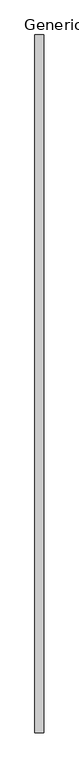
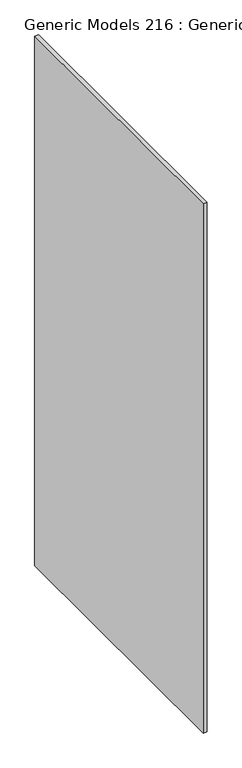
"""IFC4 building model written with IfcOpenShell, lengths in millimetres: proxy geometry, Generic Models 216 : Generic Models 1."""

from ifc_helpers import new_model, si_unit, frame, origin, place, context, project, spatial, polyline, outline, extrude, source, transform, mapped, element, save


def generic_models_216_generic_models_1_bf22bbd9(model_context):
    return source(origin(), model_context, "Body", "SweptSolid", [
        extrude(outline(polyline([(48582.2625, 1219.2), (48582.2625, 0.0), (48566.3875, 0.0), (48566.3875, 1219.2), (48582.2625, 1219.2)])), frame((0.0, 0.0, 3054.35), z_axis=(0.0, 0.0, 1.0), x_axis=(1.0, 0.0, 0.0)), (0.0, 0.0, 1.0), 2336.8),
    ])


if __name__ == "__main__":
    model = new_model("IFC4")
    model_context = context("Model", 3, world=origin())
    ifc_project = project(units=[si_unit("LENGTHUNIT", "METRE", prefix="MILLI")], contexts=[model_context])
    site = spatial("IfcSite", under=ifc_project)
    building = spatial("IfcBuilding", under=site)
    placement = place(None, origin())
    generic_models_216_generic_models_1_shape = generic_models_216_generic_models_1_bf22bbd9(model_context)
    element("IfcBuildingElementProxy", 1, Name="Generic Models 216 : Generic Models 1", ObjectType="Generic Models 216 : Generic Models 1", at=placement, inside=building, context=model_context, shape_type="MappedRepresentation", body=[
        mapped(generic_models_216_generic_models_1_shape, transform((0.0, 0.0, 0.0), x_axis=(1.0, 0.0, 0.0), y_axis=(0.0, 1.0, 0.0), z_axis=(0.0, 0.0, 1.0))),
    ])
    save(model, "model.ifc")

# Revit data of these elements
# Element 1 (IfcBuildingElementProxy, "Generic Models 216 : Generic Models 1")
#   Materials on its faces: "GYP. BD (SEE 'WALL TAG' & 'LAYER MATERIAL SCHEDULE' FOR DETAILS)"
# Materials
#   "GYP. BD (SEE 'WALL TAG' & 'LAYER MATERIAL SCHEDULE' FOR DETAILS)": class "Generic", colour RGB 237 236 233, transparency 0, Description = "Gypsum Wall Board", Cost = 0
